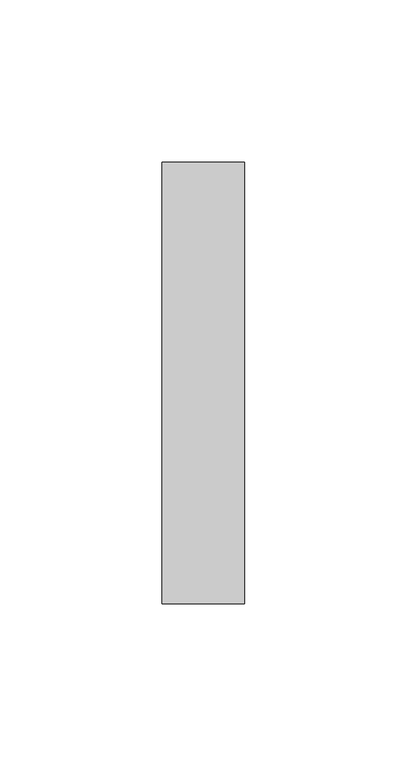
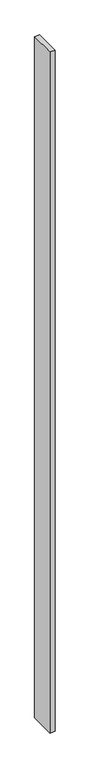
"""IFC4 building model written with IfcOpenShell, lengths in millimetres: proxy geometry, Generic Models 2:Generic Models 2:310765:Generic Models 2:310765 : Generic Models 2:Generic Models 2:310765:65 : Generic Models 2:Generic Models 2:310765:Generic Models 2:310765 : Generic Models 2:Generic Models 2:310765:300385."""

from ifc_helpers import new_model, si_unit, frame, origin, place, context, project, spatial, polyline, outline, extrude, source, transform, mapped, element, save


def generic_models_de1d64c4(model_context):
    return source(origin(), model_context, "Body", "SweptSolid", [
        extrude(outline(polyline([(578647.3117239, -568272.2400134), (578621.8863239, -568272.2400134), (578621.8863239, -568136.3050837), (578647.3117239, -568136.3050837), (578647.3117239, -568272.2400134)])), frame((0.0, 0.0, 4860.0679991), z_axis=(0.0, 0.0, 1.0), x_axis=(1.0, 0.0, 0.0)), (0.0, 0.0, 1.0), 3695.7),
    ])


if __name__ == "__main__":
    model = new_model("IFC4")
    model_context = context("Model", 3, world=origin())
    ifc_project = project(units=[si_unit("LENGTHUNIT", "METRE", prefix="MILLI")], contexts=[model_context])
    site = spatial("IfcSite", under=ifc_project)
    building = spatial("IfcBuilding", under=site)
    placement = place(None, origin())
    generic_models_shape = generic_models_de1d64c4(model_context)
    element("IfcBuildingElementProxy", 1, Name="Generic Models 2:Generic Models 2:310765:Generic Models 2:310765 : Generic Models 2:Generic Models 2:310765:65 : Generic Models 2:Generic Models 2:310765:Generic Models 2:310765 : Generic Models 2:Generic Models 2:310765:300385", ObjectType="Generic Models 2:Generic Models 2:310765:Generic Models 2:310765 : Generic Models 2:Generic Models 2:310765:65 : Generic Models 2:Generic Models 2:310765:Generic Models 2:310765 : Generic Models 2:Generic Models 2:310765:300385", at=placement, inside=building, context=model_context, shape_type="MappedRepresentation", body=[
        mapped(generic_models_shape, transform((0.0, 0.0, 0.0), x_axis=(1.0, 0.0, 0.0), y_axis=(0.0, 1.0, 0.0), z_axis=(0.0, 0.0, 1.0))),
    ])
    save(model, "model.ifc")

# Revit data of these elements
# Type "Generic Models 2:Generic Models 2:310765:Generic Models 2:310765 : Generic Models 2:Generic Models 2:310765:65 : Generic Models 2:Generic Models 2:310765:Generic Models 2:310765 : Generic Models 2:Generic Models 2:310765:300385"
#   NameOverride = "Generic Models 2:Generic Models 2:310765:Generic Models 2:310765 : Generic Models 2:Generic Models 2:310765:300385"
#   ObjectTypeOverride = "Generic Models 2:310765 : Generic Models 2:Generic Models 2:310765"
#   Reference = "Generic Models 2"
#   Tag = "300385"
# Element 1 (IfcBuildingElementProxy, "Generic Models 2:Generic Models 2:310765:Generic Models 2:310765 : Generic Models 2:Generic Models 2:310765:65 : Generic Models 2:Generic Models 2:310765:Generic Models 2:310765 : Generic Models 2:Generic Models 2:310765:300385")
#   Materials on its faces: "RIGID INSULATION AT GIRTS/JAMB - (CLASS A FLAME SPREAD)"
# Materials
#   "RIGID INSULATION AT GIRTS/JAMB - (CLASS A FLAME SPREAD)": class "Unassigned", colour RGB 205 188 106, transparency 0, Cost = 0
